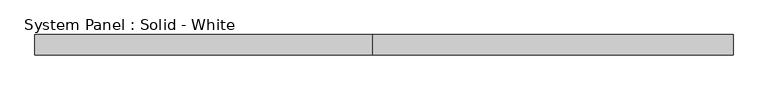
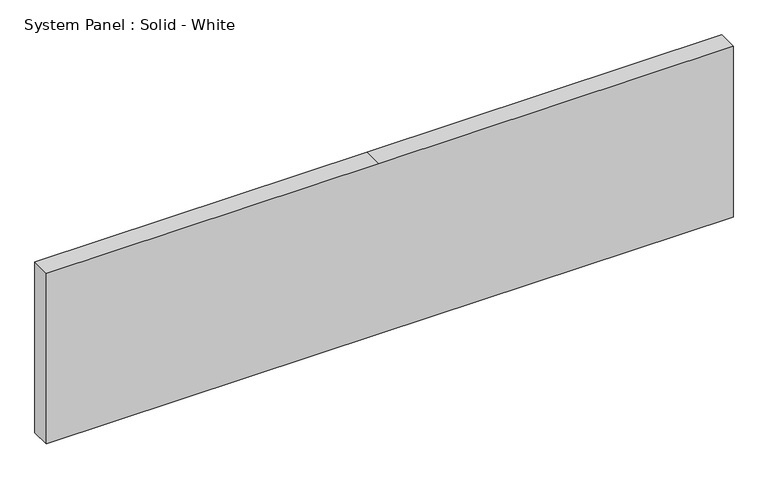
"""IFC4 building model written with IfcOpenShell, lengths in millimetres: plate geometry, System Panel : Solid - White."""

import ifcopenshell
import ifcopenshell.guid

model = None  # the IFC model being written
_history = None  # IfcOwnerHistory: only IFC2X3 demands one
_inside = {}  # id of a spatial element -> (the spatial element, [elements in it])
_under = {}  # id of a project, library or spatial element -> (it, [spatial elements below it])
_declared = {}  # id of a project -> (the project, [libraries it declares])
_typed = {}  # id of a type object -> (the type object, [elements of that type])
_made_of = {}  # id of a material, layer set ... -> (it, [elements and type objects made of it])


def new_model(schema):
    """Start an empty IFC model of exactly this schema.

    Asked for "IFC4X3", IfcOpenShell would pick the latest addendum, in which some entities
    have other attributes; the version numbers below select the first issue.
    IFC2X3 requires an IfcOwnerHistory on every rooted entity: one is made here for all.
    """
    global model, _history
    if schema == "IFC4X3":
        model = ifcopenshell.file(schema_version=(4, 3, 0, 0))
    else:
        model = ifcopenshell.file(schema=schema)
    _inside.clear()
    _under.clear()
    _declared.clear()
    _typed.clear()
    _made_of.clear()
    _history = None
    if model.schema == "IFC2X3":
        org = make("IfcOrganization", Name="unknown")
        user = make(
            "IfcPersonAndOrganization",
            ThePerson=make("IfcPerson", FamilyName="unknown"),
            TheOrganization=org,
        )
        app = make(
            "IfcApplication",
            ApplicationDeveloper=org,
            Version="unknown",
            ApplicationFullName="unknown",
            ApplicationIdentifier="unknown",
        )
        _history = make(
            "IfcOwnerHistory",
            OwningUser=user,
            OwningApplication=app,
            ChangeAction="ADDED",
            CreationDate=0,
        )
    return model


def make(cls, **values):
    """One entity of the class cls with the attributes given. An attribute that is None is left unset."""
    return model.create_entity(
        cls, **{name: value for name, value in values.items() if value is not None}
    )


def rooted(cls, **values):
    """An entity with a GlobalId (a new one), such as an element, a storey or a relation."""
    return make(cls, GlobalId=ifcopenshell.guid.new(), OwnerHistory=_history, **values)


def si_unit(unit_type, name, prefix=None):
    """IfcSIUnit, for example si_unit("LENGTHUNIT", "METRE", prefix="MILLI")."""
    return make("IfcSIUnit", UnitType=unit_type, Prefix=prefix, Name=name)


def assignment(units):
    """IfcUnitAssignment: the units of a project."""
    return None if units is None else make("IfcUnitAssignment", Units=units)


def point(xyz):
    """IfcCartesianPoint."""
    return None if xyz is None else make("IfcCartesianPoint", Coordinates=xyz)


def direction(xyz):
    """IfcDirection."""
    return None if xyz is None else make("IfcDirection", DirectionRatios=xyz)


def frame(location, z_axis=None, x_axis=None):
    """IfcAxis2Placement3D, a coordinate frame: its origin and axes. An axis left out is left unset."""
    return make(
        "IfcAxis2Placement3D",
        Location=point(location),
        Axis=direction(z_axis),
        RefDirection=direction(x_axis),
    )


def origin():
    """The frame at (0, 0, 0) with its axes left unset."""
    return frame((0.0, 0.0, 0.0))


def place(relative_to, where):
    """IfcLocalPlacement: puts the frame where relative to a parent placement (None: the world)."""
    return make(
        "IfcLocalPlacement", PlacementRelTo=relative_to, RelativePlacement=where
    )


def context(
    kind, dimensions, precision=None, world=None, true_north=None, identifier=None
):
    """IfcGeometricRepresentationContext, for example the 3D "Model" context."""
    return make(
        "IfcGeometricRepresentationContext",
        ContextIdentifier=identifier,
        ContextType=kind,
        CoordinateSpaceDimension=dimensions,
        Precision=precision,
        WorldCoordinateSystem=world,
        TrueNorth=true_north,
    )


def project(units=None, contexts=None):
    """IfcProject with its units and contexts."""
    return rooted(
        "IfcProject",
        Name="project",
        RepresentationContexts=contexts,
        UnitsInContext=assignment(units),
    )


def spatial(cls, under=None, at=None, **own):
    """A site, building, storey or space (cls), placed at a placement, below another one or the project."""
    s = rooted(cls, ObjectPlacement=at, **own)
    if under is not None:
        _under.setdefault(under.id(), (under, []))[1].append(s)
    return s


def polyline(points):
    """IfcPolyline through the points."""
    return make("IfcPolyline", Points=[point(p) for p in points])


def outline(outer, holes=None, kind="AREA"):
    """IfcArbitraryClosedProfileDef: a profile drawn as a closed curve; with holes, ...WithVoids."""
    if holes is None:
        return make("IfcArbitraryClosedProfileDef", ProfileType=kind, OuterCurve=outer)
    return make(
        "IfcArbitraryProfileDefWithVoids",
        ProfileType=kind,
        OuterCurve=outer,
        InnerCurves=holes,
    )


def extrude(swept, where, along, depth):
    """IfcExtrudedAreaSolid: the profile swept, set in the frame where, extruded along a direction by depth."""
    return make(
        "IfcExtrudedAreaSolid",
        SweptArea=swept,
        Position=where,
        ExtrudedDirection=direction(along),
        Depth=depth,
    )


def shape(context_of_items, identifier, shape_type, items):
    """IfcShapeRepresentation: the items that make up one representation, for example the "Body"."""
    return make(
        "IfcShapeRepresentation",
        ContextOfItems=context_of_items,
        RepresentationIdentifier=identifier,
        RepresentationType=shape_type,
        Items=items,
    )


def source(mapping_origin, context_of_items, identifier, shape_type, items):
    """IfcRepresentationMap: a shape defined once, which mapped items show again and again."""
    return make(
        "IfcRepresentationMap",
        MappingOrigin=mapping_origin,
        MappedRepresentation=shape(context_of_items, identifier, shape_type, items),
    )


def transform(
    local_origin,
    x_axis=None,
    y_axis=None,
    z_axis=None,
    scale=None,
    scale2=None,
    scale3=None,
    uniform=True,
):
    """IfcCartesianTransformationOperator3D, or its non-uniform kind. x_axis, y_axis, z_axis: its Axis1, 2, 3."""
    if uniform:
        return make(
            "IfcCartesianTransformationOperator3D",
            Axis1=direction(x_axis),
            Axis2=direction(y_axis),
            LocalOrigin=point(local_origin),
            Scale=scale,
            Axis3=direction(z_axis),
        )
    return make(
        "IfcCartesianTransformationOperator3DnonUniform",
        Axis1=direction(x_axis),
        Axis2=direction(y_axis),
        LocalOrigin=point(local_origin),
        Scale=scale,
        Axis3=direction(z_axis),
        Scale2=scale2,
        Scale3=scale3,
    )


def mapped(mapping_source, mapping_target):
    """IfcMappedItem: shows the shape of a source again, moved by a transform."""
    return make(
        "IfcMappedItem", MappingSource=mapping_source, MappingTarget=mapping_target
    )


def made_of(thing, what):
    """Note that an element or type object is made of a material, layer set ...; save() writes the relation."""
    if what is not None:
        _made_of.setdefault(what.id(), (what, []))[1].append(thing)
    return thing


def element(
    cls,
    number,
    at=None,
    inside=None,
    cuts=None,
    type_object=None,
    material=None,
    context=None,
    identifier="Body",
    shape_type=None,
    held_by="IfcProductDefinitionShape",
    body=None,
    shapes=None,
    **own,
):
    """One element of the class cls, such as IfcWall. Its Tag is "e" and its number.

    at: its placement. inside: the storey or other place that contains it. cuts: it is an
    opening in that element (IfcRelVoidsElement). A single representation is given by context,
    identifier, shape_type and body (its items); several are given by shapes. held_by: the class
    of the entity that holds the representations. save() writes the other relations.
    """
    e = rooted(cls, Tag="e%d" % number, ObjectPlacement=at, **own)
    if body is not None:
        shapes = [shape(context, identifier, shape_type, body)]
    if shapes is not None:
        e.Representation = make(held_by, Representations=shapes)
    if inside is not None:
        _inside.setdefault(inside.id(), (inside, []))[1].append(e)
    if cuts is not None:
        rooted(
            "IfcRelVoidsElement", RelatingBuildingElement=cuts, RelatedOpeningElement=e
        )
    if type_object is not None:
        _typed.setdefault(type_object.id(), (type_object, []))[1].append(e)
    return made_of(e, material)


def aggregate(whole, parts):
    """IfcRelAggregates: a whole, such as a stair, and the parts it consists of."""
    return rooted("IfcRelAggregates", RelatingObject=whole, RelatedObjects=parts)


def save(model, path):
    """Write the relations noted so far, then the file.

    IfcRelAggregates (storeys below a building ...), IfcRelContainedInSpatialStructure (elements
    in a storey), IfcRelDefinesByType, IfcRelAssociatesMaterial and IfcRelDeclares: one each for
    every whole, place, type object, material and project.
    """
    for whole, parts in _under.values():
        aggregate(whole, parts)
    for where, things in _inside.values():
        rooted(
            "IfcRelContainedInSpatialStructure",
            RelatedElements=things,
            RelatingStructure=where,
        )
    for kind, things in _typed.values():
        rooted("IfcRelDefinesByType", RelatedObjects=things, RelatingType=kind)
    for what, things in _made_of.values():
        rooted("IfcRelAssociatesMaterial", RelatedObjects=things, RelatingMaterial=what)
    for by, libraries in _declared.values():
        rooted("IfcRelDeclares", RelatingContext=by, RelatedDefinitions=libraries)
    model.write(path)


def system_panel_solid_white_8c86d5e4(model_context):
    return source(origin(), model_context, "Body", "SweptSolid", [
        extrude(outline(polyline([(0.0, -1099.185), (0.0, -34.925), (0.0, 1099.185), (577.85, 1099.185), (577.85, -34.925), (577.85, -1099.185), (0.0, -1099.185)])), frame((0.0, -19.05, 0.0), z_axis=(0.0, 1.0, 0.0), x_axis=(0.0, 0.0, 1.0)), (0.0, 0.0, 1.0), 63.5),
    ])


if __name__ == "__main__":
    model = new_model("IFC4")
    model_context = context("Model", 3, world=origin())
    ifc_project = project(units=[si_unit("LENGTHUNIT", "METRE", prefix="MILLI")], contexts=[model_context])
    site = spatial("IfcSite", under=ifc_project)
    building = spatial("IfcBuilding", under=site)
    placement = place(None, origin())
    system_panel_solid_white_shape = system_panel_solid_white_8c86d5e4(model_context)
    element("IfcPlate", 1, ObjectType="System Panel : Solid - White", at=placement, inside=building, context=model_context, shape_type="MappedRepresentation", body=[
        mapped(system_panel_solid_white_shape, transform((0.0, 0.0, 0.0), x_axis=(1.0, 0.0, 0.0), y_axis=(0.0, 1.0, 0.0), z_axis=(0.0, 0.0, 1.0))),
    ])
    save(model, "model.ifc")

# Revit data of these elements
# Element 1 (IfcPlate, "System Panel : Solid - White")
#   Materials on its faces: "White Panel"
# Materials
#   "White Panel": class "Unassigned", colour RGB 255 255 255, transparency 0
